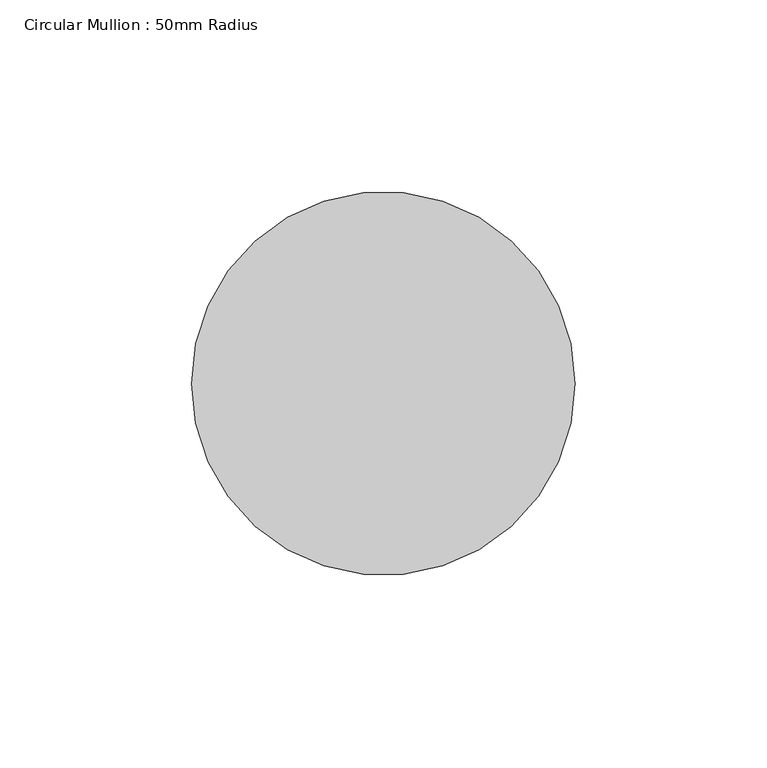
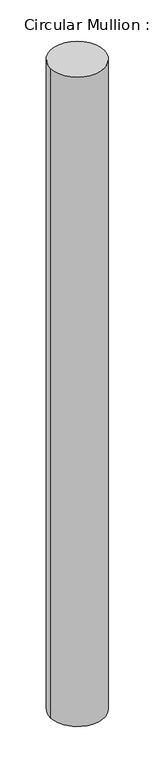
"""IFC4 building model written with IfcOpenShell, lengths in millimetres: member geometry, Circular Mullion : 50mm Radius."""

from ifc_helpers import new_model, si_unit, point, frame, origin, origin_2d, place, context, project, spatial, circle_curve, trimmed, segment, composite_curve, outline, extrude, source, transform, mapped, element, save


def circular_mullion_50mm_radius_dfee10ac(model_context):
    return source(origin(), model_context, "Body", "SweptSolid", [
        extrude(outline(composite_curve([segment(trimmed(circle_curve(origin_2d(), 50.0), [point((50.0, 0.0))], [point((-50.0, 0.0))], False, "CARTESIAN"), True, "CONTINUOUS"), segment(trimmed(circle_curve(origin_2d(), 50.0), [point((-50.0, 0.0))], [point((50.0, 0.0))], False, "CARTESIAN"), True, "CONTINUOUS")], self_intersect=False)), frame((0.0, 0.0, -1276.0779078), z_axis=(0.0, 0.0, 1.0), x_axis=(1.0, 0.0, 0.0)), (0.0, 0.0, 1.0), 1276.0779078),
    ])


if __name__ == "__main__":
    model = new_model("IFC4")
    model_context = context("Model", 3, world=origin())
    ifc_project = project(units=[si_unit("LENGTHUNIT", "METRE", prefix="MILLI")], contexts=[model_context])
    site = spatial("IfcSite", under=ifc_project)
    building = spatial("IfcBuilding", under=site)
    placement = place(None, origin())
    circular_mullion_50mm_radius_shape = circular_mullion_50mm_radius_dfee10ac(model_context)
    element("IfcMember", 1, ObjectType="Circular Mullion : 50mm Radius", at=placement, inside=building, context=model_context, shape_type="MappedRepresentation", body=[
        mapped(circular_mullion_50mm_radius_shape, transform((0.0, 0.0, 0.0), x_axis=(1.0, 0.0, 0.0), y_axis=(0.0, 1.0, 0.0), z_axis=(0.0, 0.0, 1.0))),
    ])
    save(model, "model.ifc")

# Revit data of these elements
# Type "Circular Mullion : 50mm Radius"
#   built-in parameter 1007350 = 0.164042 (stored number, unit not read)
# Element 1 (IfcMember, "Circular Mullion : 50mm Radius")
#   Materials on its faces: "Aluminium"
# Materials
#   "Aluminium": class "Metal", colour RGB 247 247 247, transparency 0, Description = "Aluminium 6061", Cost = 0
